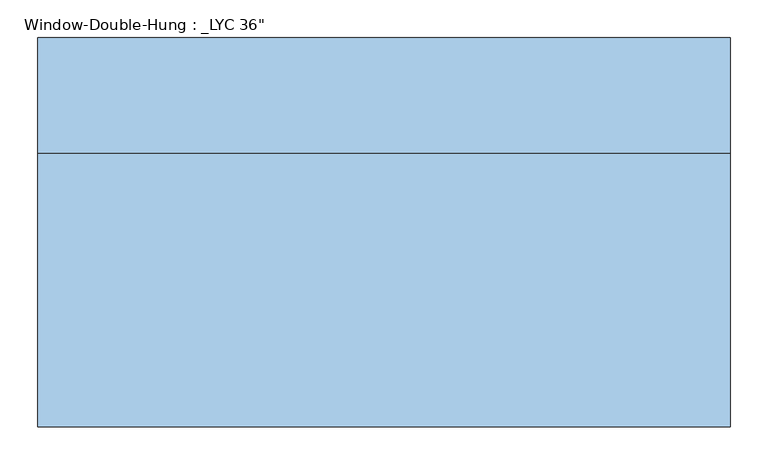
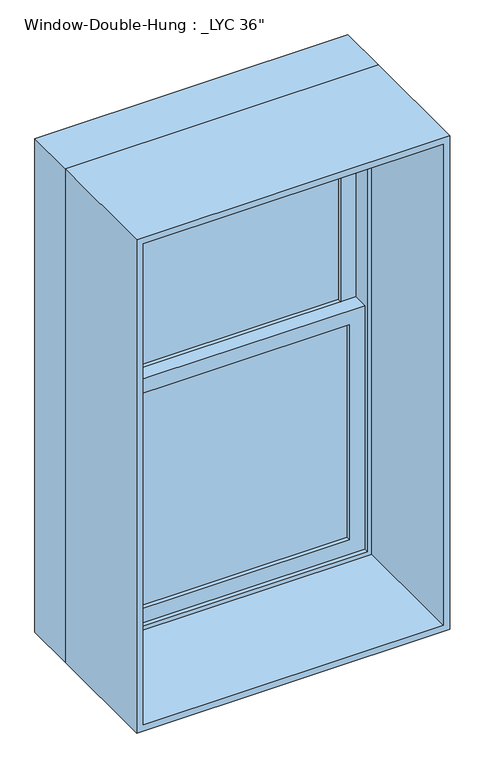
"""IFC4 building model written with IfcOpenShell, lengths in millimetres: window geometry."""

from ifc_helpers import new_model, si_unit, frame, origin, place, context, project, spatial, polyline, outline, extrude, source, transform, mapped, element, save


def window_79efe5ba(model_context):
    return source(origin(), model_context, "Body", "SweptSolid", [
        extrude(outline(polyline([(381.0, 158.75), (381.0, 152.4), (-381.0, 152.4), (-381.0, 158.75), (381.0, 158.75)])), frame((0.0, 0.0, 990.6), z_axis=(0.0, 0.0, 1.0), x_axis=(1.0, 0.0, 0.0)), (0.0, 0.0, 1.0), 663.575),
        extrude(outline(polyline([(-381.0, 146.05), (381.0, 146.05), (381.0, 139.7), (-381.0, 139.7), (-381.0, 146.05)])), frame((0.0, 0.0, 990.6), z_axis=(0.0, 0.0, 1.0), x_axis=(1.0, 0.0, 0.0)), (0.0, 0.0, 1.0), 663.575),
        extrude(outline(polyline([(381.0, 203.2), (381.0, 196.85), (-381.0, 196.85), (-381.0, 203.2), (381.0, 203.2)])), frame((0.0, 0.0, 1698.625), z_axis=(0.0, 0.0, 1.0), x_axis=(1.0, 0.0, 0.0)), (0.0, 0.0, 1.0), 663.575),
        extrude(outline(polyline([(-381.0, 190.5), (381.0, 190.5), (381.0, 184.15), (-381.0, 184.15), (-381.0, 190.5)])), frame((0.0, 0.0, 1698.625), z_axis=(0.0, 0.0, 1.0), x_axis=(1.0, 0.0, 0.0)), (0.0, 0.0, 1.0), 663.575),
        extrude(outline(polyline([(1698.625, -425.45), (946.15, -425.45), (946.15, 425.45), (1698.625, 425.45), (1698.625, -425.45)]), holes=[polyline([(1654.175, 381.0), (990.6, 381.0), (990.6, -381.0), (1654.175, -381.0), (1654.175, 381.0)])]), frame((0.0, 127.0, 0.0), z_axis=(0.0, 1.0, 0.0), x_axis=(0.0, 0.0, 1.0)), (0.0, 0.0, 1.0), 44.45),
        extrude(outline(polyline([(2406.65, -425.45), (1654.175, -425.45), (1654.175, 425.45), (2406.65, 425.45), (2406.65, -425.45)]), holes=[polyline([(2362.2, 381.0), (1698.625, 381.0), (1698.625, -381.0), (2362.2, -381.0), (2362.2, 381.0)])]), frame((0.0, 171.45, 0.0), z_axis=(0.0, 1.0, 0.0), x_axis=(0.0, 0.0, 1.0)), (0.0, 0.0, 1.0), 44.45),
        extrude(outline(polyline([(2438.4, -457.2), (914.4, -457.2), (914.4, 457.2), (2438.4, 457.2), (2438.4, -457.2)]), holes=[polyline([(2406.65, 425.45), (946.15, 425.45), (946.15, -425.45), (2406.65, -425.45), (2406.65, 425.45)])]), frame((0.0, 114.3, 0.0), z_axis=(0.0, 1.0, 0.0), x_axis=(0.0, 0.0, 1.0)), (0.0, 0.0, 1.0), 152.4),
        extrude(outline(polyline([(2438.4, 457.2), (2438.4, -457.2), (914.4, -457.2), (914.4, 457.2), (2438.4, 457.2)]), holes=[polyline([(2419.35, 438.15), (933.45, 438.15), (933.45, -438.15), (2419.35, -438.15), (2419.35, 438.15)])]), frame((0.0, -247.65, 0.0), z_axis=(0.0, 1.0, 0.0), x_axis=(0.0, 0.0, 1.0)), (0.0, 0.0, 1.0), 361.95),
    ])


if __name__ == "__main__":
    model = new_model("IFC4")
    model_context = context("Model", 3, world=origin())
    ifc_project = project(units=[si_unit("LENGTHUNIT", "METRE", prefix="MILLI")], contexts=[model_context])
    site = spatial("IfcSite", under=ifc_project)
    building = spatial("IfcBuilding", under=site)
    placement = place(None, origin())
    window_shape = window_79efe5ba(model_context)
    element("IfcWindow", 1, ObjectType="Window-Double-Hung : _LYC 36\"", at=placement, inside=building, context=model_context, shape_type="MappedRepresentation", body=[
        mapped(window_shape, transform((0.0, 0.0, 0.0), x_axis=(1.0, 0.0, 0.0), y_axis=(0.0, 1.0, 0.0), z_axis=(0.0, 0.0, 1.0))),
    ])
    save(model, "model.ifc")

# Revit data of these elements
# Type "Window-Double-Hung : _LYC 36\""
#   Type Mark = "20"
#   Fire Rating = "0.5h"
#   Assembly Code = "B2020100"
#   Wall Thickness [instance default] = 0' - 6"
#   Visual Light Transmittance = 0.9
#   Thermal Resistance (R) = 1.8146 (h·ft²·°F)/BTU
#   Solar Heat Gain Coefficient = 0.78
#   Rough Width = 3' - 0 1/2"
#   Rough Height = 5' - 0 1/2"
#   Muntin Width = 2' - 6"
#   Muntin Height = 2' - 2 1/8"
#   Interior Wall Closure [instance default] = 0' - 1 1/2"
#   Heat Transfer Coefficient (U) = 0.6496 BTU/(h·ft²·°F)
#   Frame Extension [instance default] = 0' - 2"
#   Exterior Wall Closure [instance default] = 0' - 0 1/2"
#   Extension Jamb [instance default] = 0' - 0 3/4"
#   Height = 5' - 0"
#   Width = 3' - 0"
#   Window Inset [instance default] = 0' - 0 3/4"
#   Top Muntin Visibility = yes
#   Interior Trim Visibility [instance default] = yes
#   Indicator Visibility [instance default] = yes
#   Exterior Trim Visibility [instance default] = yes
#   Extension Jamb Visibility [instance default] = yes
#   Define Thermal Properties by = 1
#   Bottom Muntin Visibility = yes
#   Muntin Pattern = Muntin Pattern_2x2 : Muntin Pattern_2x2
#   Interior Trim Material = Wood - Stained
#   Interior Trim = Trim-Window-Interior-Flat : Picture Frame
#   Interior Frame Material = Wood - Stained
#   Glass Panel Material = Glass
#   Exterior Trim Material = Clad - White
#   Exterior Trim = Trim-Window-Exterior-Flat : with Sill
#   Exterior Frame Material = Clad - White
#   Construction Type Id = ""
#   Wall Closure = (empty or 0)
#   Analytic Construction = (empty or 0)
# Element 1 (IfcWindow, "Window-Double-Hung : _LYC 36\"")
#   Wall Thickness = 1' - 7 1/2"
#   Extension Jamb = 1' - 2 1/4"
#   Materials on its faces: "Wood - Stained", "Glass", "Clad - White"
# Materials
#   "Wood - Stained": class "Wood", colour RGB 224 178 126, transparency 0, Cost = 0
#   "Glass": class "Unassigned", colour RGB 0 128 192, transparency 0.75
#   "Clad - White": class "Wood", colour RGB 242 242 238, transparency 0, Cost = 0
